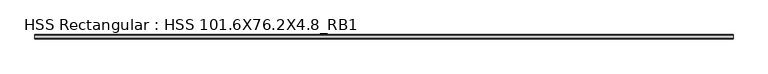
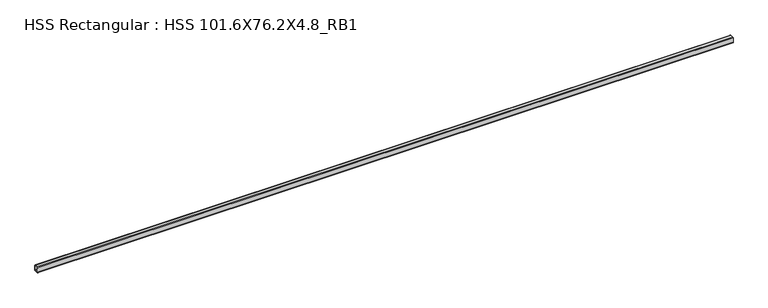
"""IFC4 building model written with IfcOpenShell, lengths in millimetres: beam geometry, HSS Rectangular : HSS 101.6X76.2X4.8_RB1."""

import ifcopenshell
import ifcopenshell.guid

model = None  # the IFC model being written
_history = None  # IfcOwnerHistory: only IFC2X3 demands one
_inside = {}  # id of a spatial element -> (the spatial element, [elements in it])
_under = {}  # id of a project, library or spatial element -> (it, [spatial elements below it])
_declared = {}  # id of a project -> (the project, [libraries it declares])
_typed = {}  # id of a type object -> (the type object, [elements of that type])
_made_of = {}  # id of a material, layer set ... -> (it, [elements and type objects made of it])


def new_model(schema):
    """Start an empty IFC model of exactly this schema.

    Asked for "IFC4X3", IfcOpenShell would pick the latest addendum, in which some entities
    have other attributes; the version numbers below select the first issue.
    IFC2X3 requires an IfcOwnerHistory on every rooted entity: one is made here for all.
    """
    global model, _history
    if schema == "IFC4X3":
        model = ifcopenshell.file(schema_version=(4, 3, 0, 0))
    else:
        model = ifcopenshell.file(schema=schema)
    _inside.clear()
    _under.clear()
    _declared.clear()
    _typed.clear()
    _made_of.clear()
    _history = None
    if model.schema == "IFC2X3":
        org = make("IfcOrganization", Name="unknown")
        user = make(
            "IfcPersonAndOrganization",
            ThePerson=make("IfcPerson", FamilyName="unknown"),
            TheOrganization=org,
        )
        app = make(
            "IfcApplication",
            ApplicationDeveloper=org,
            Version="unknown",
            ApplicationFullName="unknown",
            ApplicationIdentifier="unknown",
        )
        _history = make(
            "IfcOwnerHistory",
            OwningUser=user,
            OwningApplication=app,
            ChangeAction="ADDED",
            CreationDate=0,
        )
    return model


def make(cls, **values):
    """One entity of the class cls with the attributes given. An attribute that is None is left unset."""
    return model.create_entity(
        cls, **{name: value for name, value in values.items() if value is not None}
    )


def rooted(cls, **values):
    """An entity with a GlobalId (a new one), such as an element, a storey or a relation."""
    return make(cls, GlobalId=ifcopenshell.guid.new(), OwnerHistory=_history, **values)


def si_unit(unit_type, name, prefix=None):
    """IfcSIUnit, for example si_unit("LENGTHUNIT", "METRE", prefix="MILLI")."""
    return make("IfcSIUnit", UnitType=unit_type, Prefix=prefix, Name=name)


def assignment(units):
    """IfcUnitAssignment: the units of a project."""
    return None if units is None else make("IfcUnitAssignment", Units=units)


def point(xyz):
    """IfcCartesianPoint."""
    return None if xyz is None else make("IfcCartesianPoint", Coordinates=xyz)


def direction(xyz):
    """IfcDirection."""
    return None if xyz is None else make("IfcDirection", DirectionRatios=xyz)


def frame(location, z_axis=None, x_axis=None):
    """IfcAxis2Placement3D, a coordinate frame: its origin and axes. An axis left out is left unset."""
    return make(
        "IfcAxis2Placement3D",
        Location=point(location),
        Axis=direction(z_axis),
        RefDirection=direction(x_axis),
    )


def frame_2d(location, x_axis=None):
    """IfcAxis2Placement2D, a coordinate frame in the plane: its origin and x axis."""
    return make(
        "IfcAxis2Placement2D", Location=point(location), RefDirection=direction(x_axis)
    )


def origin():
    """The frame at (0, 0, 0) with its axes left unset."""
    return frame((0.0, 0.0, 0.0))


def place(relative_to, where):
    """IfcLocalPlacement: puts the frame where relative to a parent placement (None: the world)."""
    return make(
        "IfcLocalPlacement", PlacementRelTo=relative_to, RelativePlacement=where
    )


def context(
    kind, dimensions, precision=None, world=None, true_north=None, identifier=None
):
    """IfcGeometricRepresentationContext, for example the 3D "Model" context."""
    return make(
        "IfcGeometricRepresentationContext",
        ContextIdentifier=identifier,
        ContextType=kind,
        CoordinateSpaceDimension=dimensions,
        Precision=precision,
        WorldCoordinateSystem=world,
        TrueNorth=true_north,
    )


def project(units=None, contexts=None):
    """IfcProject with its units and contexts."""
    return rooted(
        "IfcProject",
        Name="project",
        RepresentationContexts=contexts,
        UnitsInContext=assignment(units),
    )


def spatial(cls, under=None, at=None, **own):
    """A site, building, storey or space (cls), placed at a placement, below another one or the project."""
    s = rooted(cls, ObjectPlacement=at, **own)
    if under is not None:
        _under.setdefault(under.id(), (under, []))[1].append(s)
    return s


def polyline(points):
    """IfcPolyline through the points."""
    return make("IfcPolyline", Points=[point(p) for p in points])


def circle_curve(where, radius):
    """IfcCircle in the frame where."""
    return make("IfcCircle", Position=where, Radius=radius)


def trimmed(basis, trim1, trim2, sense, master):
    """IfcTrimmedCurve: the piece of a basis curve between two trims."""
    return make(
        "IfcTrimmedCurve",
        BasisCurve=basis,
        Trim1=trim1,
        Trim2=trim2,
        SenseAgreement=sense,
        MasterRepresentation=master,
    )


def segment(curve, same_sense, transition):
    """IfcCompositeCurveSegment."""
    return make(
        "IfcCompositeCurveSegment",
        Transition=transition,
        SameSense=same_sense,
        ParentCurve=curve,
    )


def composite_curve(segments, self_intersect=None):
    """IfcCompositeCurve: segments joined end to end."""
    return make("IfcCompositeCurve", Segments=segments, SelfIntersect=self_intersect)


def outline(outer, holes=None, kind="AREA"):
    """IfcArbitraryClosedProfileDef: a profile drawn as a closed curve; with holes, ...WithVoids."""
    if holes is None:
        return make("IfcArbitraryClosedProfileDef", ProfileType=kind, OuterCurve=outer)
    return make(
        "IfcArbitraryProfileDefWithVoids",
        ProfileType=kind,
        OuterCurve=outer,
        InnerCurves=holes,
    )


def extrude(swept, where, along, depth):
    """IfcExtrudedAreaSolid: the profile swept, set in the frame where, extruded along a direction by depth."""
    return make(
        "IfcExtrudedAreaSolid",
        SweptArea=swept,
        Position=where,
        ExtrudedDirection=direction(along),
        Depth=depth,
    )


def shape(context_of_items, identifier, shape_type, items):
    """IfcShapeRepresentation: the items that make up one representation, for example the "Body"."""
    return make(
        "IfcShapeRepresentation",
        ContextOfItems=context_of_items,
        RepresentationIdentifier=identifier,
        RepresentationType=shape_type,
        Items=items,
    )


def source(mapping_origin, context_of_items, identifier, shape_type, items):
    """IfcRepresentationMap: a shape defined once, which mapped items show again and again."""
    return make(
        "IfcRepresentationMap",
        MappingOrigin=mapping_origin,
        MappedRepresentation=shape(context_of_items, identifier, shape_type, items),
    )


def transform(
    local_origin,
    x_axis=None,
    y_axis=None,
    z_axis=None,
    scale=None,
    scale2=None,
    scale3=None,
    uniform=True,
):
    """IfcCartesianTransformationOperator3D, or its non-uniform kind. x_axis, y_axis, z_axis: its Axis1, 2, 3."""
    if uniform:
        return make(
            "IfcCartesianTransformationOperator3D",
            Axis1=direction(x_axis),
            Axis2=direction(y_axis),
            LocalOrigin=point(local_origin),
            Scale=scale,
            Axis3=direction(z_axis),
        )
    return make(
        "IfcCartesianTransformationOperator3DnonUniform",
        Axis1=direction(x_axis),
        Axis2=direction(y_axis),
        LocalOrigin=point(local_origin),
        Scale=scale,
        Axis3=direction(z_axis),
        Scale2=scale2,
        Scale3=scale3,
    )


def mapped(mapping_source, mapping_target):
    """IfcMappedItem: shows the shape of a source again, moved by a transform."""
    return make(
        "IfcMappedItem", MappingSource=mapping_source, MappingTarget=mapping_target
    )


def made_of(thing, what):
    """Note that an element or type object is made of a material, layer set ...; save() writes the relation."""
    if what is not None:
        _made_of.setdefault(what.id(), (what, []))[1].append(thing)
    return thing


def element(
    cls,
    number,
    at=None,
    inside=None,
    cuts=None,
    type_object=None,
    material=None,
    context=None,
    identifier="Body",
    shape_type=None,
    held_by="IfcProductDefinitionShape",
    body=None,
    shapes=None,
    **own,
):
    """One element of the class cls, such as IfcWall. Its Tag is "e" and its number.

    at: its placement. inside: the storey or other place that contains it. cuts: it is an
    opening in that element (IfcRelVoidsElement). A single representation is given by context,
    identifier, shape_type and body (its items); several are given by shapes. held_by: the class
    of the entity that holds the representations. save() writes the other relations.
    """
    e = rooted(cls, Tag="e%d" % number, ObjectPlacement=at, **own)
    if body is not None:
        shapes = [shape(context, identifier, shape_type, body)]
    if shapes is not None:
        e.Representation = make(held_by, Representations=shapes)
    if inside is not None:
        _inside.setdefault(inside.id(), (inside, []))[1].append(e)
    if cuts is not None:
        rooted(
            "IfcRelVoidsElement", RelatingBuildingElement=cuts, RelatedOpeningElement=e
        )
    if type_object is not None:
        _typed.setdefault(type_object.id(), (type_object, []))[1].append(e)
    return made_of(e, material)


def aggregate(whole, parts):
    """IfcRelAggregates: a whole, such as a stair, and the parts it consists of."""
    return rooted("IfcRelAggregates", RelatingObject=whole, RelatedObjects=parts)


def save(model, path):
    """Write the relations noted so far, then the file.

    IfcRelAggregates (storeys below a building ...), IfcRelContainedInSpatialStructure (elements
    in a storey), IfcRelDefinesByType, IfcRelAssociatesMaterial and IfcRelDeclares: one each for
    every whole, place, type object, material and project.
    """
    for whole, parts in _under.values():
        aggregate(whole, parts)
    for where, things in _inside.values():
        rooted(
            "IfcRelContainedInSpatialStructure",
            RelatedElements=things,
            RelatingStructure=where,
        )
    for kind, things in _typed.values():
        rooted("IfcRelDefinesByType", RelatedObjects=things, RelatingType=kind)
    for what, things in _made_of.values():
        rooted("IfcRelAssociatesMaterial", RelatedObjects=things, RelatingMaterial=what)
    for by, libraries in _declared.values():
        rooted("IfcRelDeclares", RelatingContext=by, RelatedDefinitions=libraries)
    model.write(path)


def hss_rectangular_hss_101_6x76_2x4_8_rb1_3335c383(model_context):
    return source(origin(), model_context, "Body", "SweptSolid", [
        extrude(outline(composite_curve([segment(trimmed(circle_curve(frame_2d((-28.575, 41.275)), 9.525), [point((-38.1, 41.275))], [point((-28.575, 50.8))], False, "CARTESIAN"), True, "CONTINUOUS"), segment(polyline([(-28.575, 50.8), (28.575, 50.8)]), True, "CONTINUOUS"), segment(trimmed(circle_curve(frame_2d((28.575, 41.275)), 9.525), [point((28.575, 50.8))], [point((38.1, 41.275))], False, "CARTESIAN"), True, "CONTINUOUS"), segment(polyline([(38.1, 41.275), (38.1, -41.275)]), True, "CONTINUOUS"), segment(trimmed(circle_curve(frame_2d((28.575, -41.275)), 9.525), [point((38.1, -41.275))], [point((28.575, -50.8))], False, "CARTESIAN"), True, "CONTINUOUS"), segment(polyline([(28.575, -50.8), (-28.575, -50.8)]), True, "CONTINUOUS"), segment(trimmed(circle_curve(frame_2d((-28.575, -41.275)), 9.525), [point((-28.575, -50.8))], [point((-38.1, -41.275))], False, "CARTESIAN"), True, "CONTINUOUS"), segment(polyline([(-38.1, -41.275), (-38.1, 41.275)]), True, "CONTINUOUS")], self_intersect=False), holes=[composite_curve([segment(polyline([(28.575, 46.0375), (-28.575, 46.0375)]), True, "CONTINUOUS"), segment(trimmed(circle_curve(frame_2d((-28.575, 41.275)), 4.7625), [point((-28.575, 46.0375))], [point((-33.3375, 41.275))], True, "CARTESIAN"), True, "CONTINUOUS"), segment(polyline([(-33.3375, 41.275), (-33.3375, -41.275)]), True, "CONTINUOUS"), segment(trimmed(circle_curve(frame_2d((-28.575, -41.275)), 4.7625), [point((-33.3375, -41.275))], [point((-28.575, -46.0375))], True, "CARTESIAN"), True, "CONTINUOUS"), segment(polyline([(-28.575, -46.0375), (28.575, -46.0375)]), True, "CONTINUOUS"), segment(trimmed(circle_curve(frame_2d((28.575, -41.275)), 4.7625), [point((28.575, -46.0375))], [point((33.3375, -41.275))], True, "CARTESIAN"), True, "CONTINUOUS"), segment(polyline([(33.3375, -41.275), (33.3375, 41.275)]), True, "CONTINUOUS"), segment(trimmed(circle_curve(frame_2d((28.575, 41.275)), 4.7625), [point((33.3375, 41.275))], [point((28.575, 46.0375))], True, "CARTESIAN"), True, "CONTINUOUS")], self_intersect=False)]), frame((-7457.3609994, 0.0, 0.0), z_axis=(1.0, 0.0, 0.0), x_axis=(0.0, 1.0, 0.0)), (0.0, 0.0, 1.0), 11995.4609994),
    ])


if __name__ == "__main__":
    model = new_model("IFC4")
    model_context = context("Model", 3, world=origin())
    ifc_project = project(units=[si_unit("LENGTHUNIT", "METRE", prefix="MILLI")], contexts=[model_context])
    site = spatial("IfcSite", under=ifc_project)
    building = spatial("IfcBuilding", under=site)
    placement = place(None, origin())
    hss_rectangular_hss_101_6x76_2x4_8_rb1_shape = hss_rectangular_hss_101_6x76_2x4_8_rb1_3335c383(model_context)
    element("IfcBeam", 1, ObjectType="HSS Rectangular : HSS 101.6X76.2X4.8_RB1", at=placement, inside=building, context=model_context, shape_type="MappedRepresentation", body=[
        mapped(hss_rectangular_hss_101_6x76_2x4_8_rb1_shape, transform((0.0, 0.0, 0.0), x_axis=(1.0, 0.0, 0.0), y_axis=(0.0, 1.0, 0.0), z_axis=(0.0, 0.0, 1.0))),
    ])
    save(model, "model.ifc")

# Revit data of these elements
# Type "HSS Rectangular : HSS 101.6X76.2X4.8_RB1"
#   Section Name Key = "HSS 4X3X3/16"
#   Assembly Code = "B10"
#   Width = 7.62 cm
#   Wall Nominal Thickness = 0.4763 cm
#   Wall Design Thickness = 0.442 cm
#   Torsional Moment of Inertia = 260.561 cm⁴
#   Torsional Modulus = 61.2876 cm³
#   Section Area = 14.4516 cm²
#   Plastic Modulus weak axis = 40.3122 cm³
#   Plastic Modulus strong axis = 49.1612 cm³
#   Perimeter = 0.881482 m²/m
#   Outer Fillet = 0.9525 cm
#   Nominal Weight = 12.1285 kgf/m
#   Moment of Inertia weak axis = 131.529 cm⁴
#   Moment of Inertia strong axis = 205.202 cm⁴
#   Inner Fillet = 0.4763 cm
#   Height = 10.16 cm
#   Elastic Modulus weak axis = 34.4128 cm³
#   Elastic Modulus strong axis = 40.476 cm³
#   Centroid Vertical = 5.08 cm
#   Centroid Horizontal = 3.81 cm
#   Length [instance default] = 1524 mm
#   Structural Material [instance default] = Steel ASTM A500, Grade B, Rectangular and Square
#   Principal Axes Angle = 0
# Element 1 (IfcBeam, "HSS Rectangular : HSS 101.6X76.2X4.8_RB1")
#   Structural Material = Steel ASTM A992
#   Materials on its faces: "Steel ASTM A992"
# Materials
#   "Steel ASTM A500, Grade B, Rectangular and Square": class "Metal", colour RGB 199 199 199, transparency 0, Description = "Carbon steel", Cost = 0
#   "Steel ASTM A992": class "Metal", colour RGB 199 199 199, transparency 0, Description = "Structural steel 50ksi", Cost = 0
